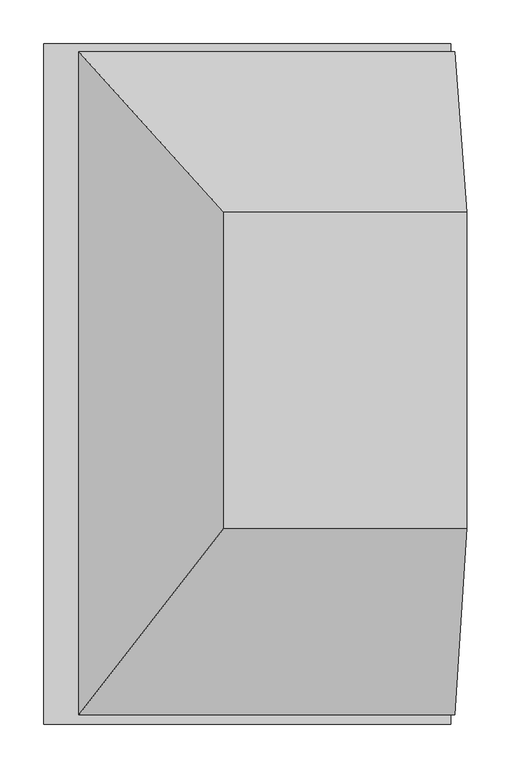
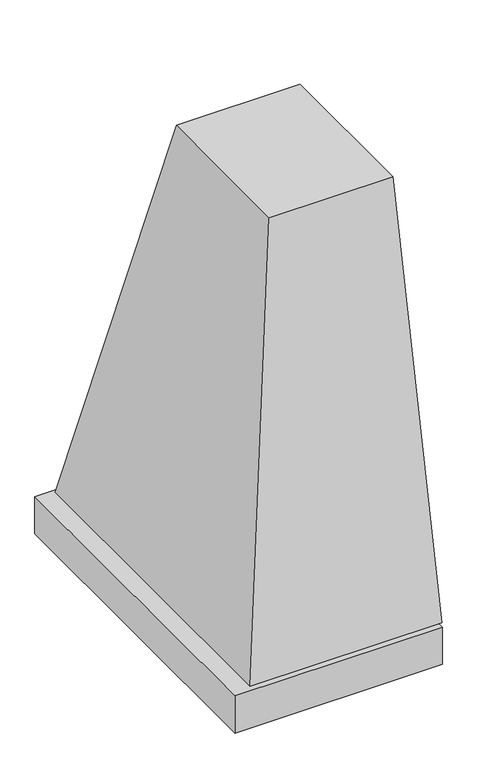
"""IFC4 building model written with IfcOpenShell, lengths in millimetres: furniture geometry, Ketichen Vent hood : Ketichen Vent hood."""

from ifc_helpers import new_model, si_unit, frame, origin, place, context, project, spatial, polyline, outline, extrude, faceted_brep, source, transform, mapped, element, save


def furniture_ccfc35a6(model_context):
    return source(origin(), model_context, "Body", "SolidModel", [
        faceted_brep([(7897.8125, 10974.8152257, 1807.7960834), (7897.8125, 11736.8152257, 1807.7960834), (8329.6125, 11736.8152257, 1807.7960834), (8329.6125, 10974.8152257, 1807.7960834), (8064.5, 11189.3086459, 2735.9332092), (8343.9, 11189.3086459, 2735.9332092), (8343.9, 11552.2193967, 2735.9332092), (8064.5, 11552.2193967, 2735.9332092)], [[[0, 1, 2, 3]], [[4, 5, 6, 7]], [[5, 4, 0, 3]], [[6, 5, 3, 2]], [[7, 6, 2, 1]], [[4, 7, 1, 0]]]),
        extrude(outline(polyline([(7857.2605033, 11746.0518595), (8325.0675324, 11746.0518595), (8325.0675324, 10963.7027257), (7857.2605033, 10963.7027257), (7857.2605033, 11746.0518595)])), frame((0.0, 0.0, 1717.1109274), z_axis=(0.0, 0.0, 1.0), x_axis=(1.0, 0.0, 0.0)), (0.0, 0.0, 1.0), 88.6699303),
    ])


if __name__ == "__main__":
    model = new_model("IFC4")
    model_context = context("Model", 3, world=origin())
    ifc_project = project(units=[si_unit("LENGTHUNIT", "METRE", prefix="MILLI")], contexts=[model_context])
    site = spatial("IfcSite", under=ifc_project)
    building = spatial("IfcBuilding", under=site)
    placement = place(None, origin())
    furniture_shape = furniture_ccfc35a6(model_context)
    element("IfcFurniture", 1, ObjectType="Ketichen Vent hood : Ketichen Vent hood", at=placement, inside=building, context=model_context, shape_type="MappedRepresentation", body=[
        mapped(furniture_shape, transform((0.0, 0.0, 0.0), x_axis=(1.0, 0.0, 0.0), y_axis=(0.0, 1.0, 0.0), z_axis=(0.0, 0.0, 1.0))),
    ])
    save(model, "model.ifc")

# Revit data of these elements
# Type "Ketichen Vent hood : Ketichen Vent hood"
#   COBie.Type = no
# Element 1 (IfcFurniture, "Ketichen Vent hood : Ketichen Vent hood")
#   Materials on its faces: "Corian - Dusk"
# Materials
#   "Corian - Dusk": class "Plastic", colour RGB 75 95 146, transparency 0, Manufacturer = "Corning", Cost = 0
